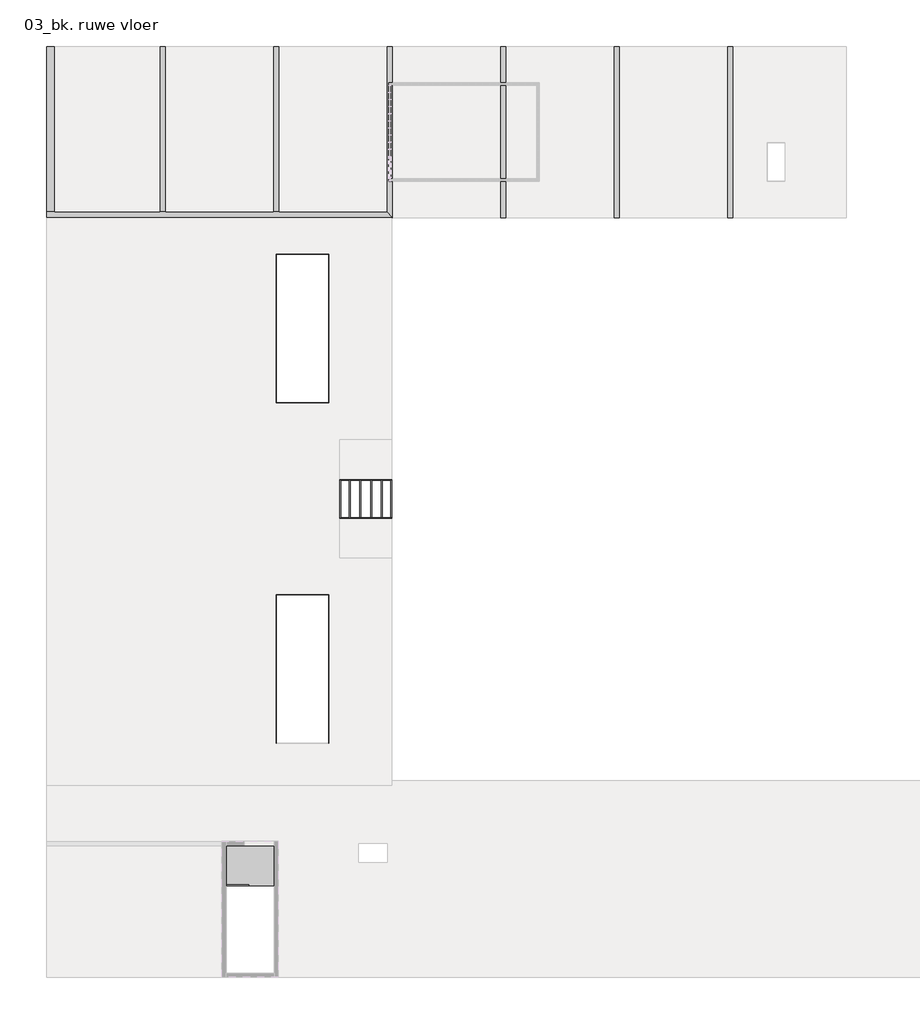
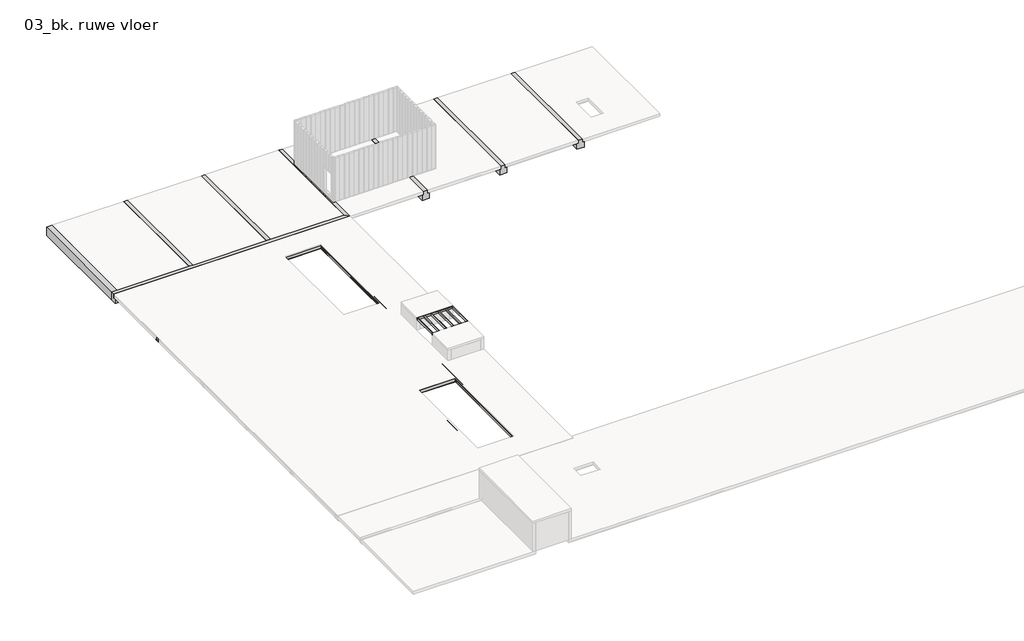
# One storey, part 9 of 9: 26 beams, 1 proxy.
"""IFC4 building model written with IfcOpenShell, lengths in millimetres."""

import ifcopenshell
import ifcopenshell.guid

model = None  # the IFC model being written
_history = None  # IfcOwnerHistory: only IFC2X3 demands one
_inside = {}  # id of a spatial element -> (the spatial element, [elements in it])
_under = {}  # id of a project, library or spatial element -> (it, [spatial elements below it])
_declared = {}  # id of a project -> (the project, [libraries it declares])
_typed = {}  # id of a type object -> (the type object, [elements of that type])
_made_of = {}  # id of a material, layer set ... -> (it, [elements and type objects made of it])


def new_model(schema):
    """Start an empty IFC model of exactly this schema.

    Asked for "IFC4X3", IfcOpenShell would pick the latest addendum, in which some entities
    have other attributes; the version numbers below select the first issue.
    IFC2X3 requires an IfcOwnerHistory on every rooted entity: one is made here for all.
    """
    global model, _history
    if schema == "IFC4X3":
        model = ifcopenshell.file(schema_version=(4, 3, 0, 0))
    else:
        model = ifcopenshell.file(schema=schema)
    _inside.clear()
    _under.clear()
    _declared.clear()
    _typed.clear()
    _made_of.clear()
    _history = None
    if model.schema == "IFC2X3":
        org = make("IfcOrganization", Name="unknown")
        user = make(
            "IfcPersonAndOrganization",
            ThePerson=make("IfcPerson", FamilyName="unknown"),
            TheOrganization=org,
        )
        app = make(
            "IfcApplication",
            ApplicationDeveloper=org,
            Version="unknown",
            ApplicationFullName="unknown",
            ApplicationIdentifier="unknown",
        )
        _history = make(
            "IfcOwnerHistory",
            OwningUser=user,
            OwningApplication=app,
            ChangeAction="ADDED",
            CreationDate=0,
        )
    return model


def make(cls, **values):
    """One entity of the class cls with the attributes given. An attribute that is None is left unset."""
    return model.create_entity(
        cls, **{name: value for name, value in values.items() if value is not None}
    )


def rooted(cls, **values):
    """An entity with a GlobalId (a new one), such as an element, a storey or a relation."""
    return make(cls, GlobalId=ifcopenshell.guid.new(), OwnerHistory=_history, **values)


def si_unit(unit_type, name, prefix=None):
    """IfcSIUnit, for example si_unit("LENGTHUNIT", "METRE", prefix="MILLI")."""
    return make("IfcSIUnit", UnitType=unit_type, Prefix=prefix, Name=name)


def assignment(units):
    """IfcUnitAssignment: the units of a project."""
    return None if units is None else make("IfcUnitAssignment", Units=units)


def point(xyz):
    """IfcCartesianPoint."""
    return None if xyz is None else make("IfcCartesianPoint", Coordinates=xyz)


def direction(xyz):
    """IfcDirection."""
    return None if xyz is None else make("IfcDirection", DirectionRatios=xyz)


def frame(location, z_axis=None, x_axis=None):
    """IfcAxis2Placement3D, a coordinate frame: its origin and axes. An axis left out is left unset."""
    return make(
        "IfcAxis2Placement3D",
        Location=point(location),
        Axis=direction(z_axis),
        RefDirection=direction(x_axis),
    )


def frame_2d(location, x_axis=None):
    """IfcAxis2Placement2D, a coordinate frame in the plane: its origin and x axis."""
    return make(
        "IfcAxis2Placement2D", Location=point(location), RefDirection=direction(x_axis)
    )


def origin():
    """The frame at (0, 0, 0) with its axes left unset."""
    return frame((0.0, 0.0, 0.0))


def place(relative_to, where):
    """IfcLocalPlacement: puts the frame where relative to a parent placement (None: the world)."""
    return make(
        "IfcLocalPlacement", PlacementRelTo=relative_to, RelativePlacement=where
    )


def context(
    kind, dimensions, precision=None, world=None, true_north=None, identifier=None
):
    """IfcGeometricRepresentationContext, for example the 3D "Model" context."""
    return make(
        "IfcGeometricRepresentationContext",
        ContextIdentifier=identifier,
        ContextType=kind,
        CoordinateSpaceDimension=dimensions,
        Precision=precision,
        WorldCoordinateSystem=world,
        TrueNorth=true_north,
    )


def project(units=None, contexts=None):
    """IfcProject with its units and contexts."""
    return rooted(
        "IfcProject",
        Name="project",
        RepresentationContexts=contexts,
        UnitsInContext=assignment(units),
    )


def spatial(cls, under=None, at=None, **own):
    """A site, building, storey or space (cls), placed at a placement, below another one or the project."""
    s = rooted(cls, ObjectPlacement=at, **own)
    if under is not None:
        _under.setdefault(under.id(), (under, []))[1].append(s)
    return s


def polyline(points):
    """IfcPolyline through the points."""
    return make("IfcPolyline", Points=[point(p) for p in points])


def circle_curve(where, radius):
    """IfcCircle in the frame where."""
    return make("IfcCircle", Position=where, Radius=radius)


def trimmed(basis, trim1, trim2, sense, master):
    """IfcTrimmedCurve: the piece of a basis curve between two trims."""
    return make(
        "IfcTrimmedCurve",
        BasisCurve=basis,
        Trim1=trim1,
        Trim2=trim2,
        SenseAgreement=sense,
        MasterRepresentation=master,
    )


def segment(curve, same_sense, transition):
    """IfcCompositeCurveSegment."""
    return make(
        "IfcCompositeCurveSegment",
        Transition=transition,
        SameSense=same_sense,
        ParentCurve=curve,
    )


def composite_curve(segments, self_intersect=None):
    """IfcCompositeCurve: segments joined end to end."""
    return make("IfcCompositeCurve", Segments=segments, SelfIntersect=self_intersect)


def outline(outer, holes=None, kind="AREA"):
    """IfcArbitraryClosedProfileDef: a profile drawn as a closed curve; with holes, ...WithVoids."""
    if holes is None:
        return make("IfcArbitraryClosedProfileDef", ProfileType=kind, OuterCurve=outer)
    return make(
        "IfcArbitraryProfileDefWithVoids",
        ProfileType=kind,
        OuterCurve=outer,
        InnerCurves=holes,
    )


def extrude(swept, where, along, depth):
    """IfcExtrudedAreaSolid: the profile swept, set in the frame where, extruded along a direction by depth."""
    return make(
        "IfcExtrudedAreaSolid",
        SweptArea=swept,
        Position=where,
        ExtrudedDirection=direction(along),
        Depth=depth,
    )


def faces_of(points, faces, orient=None, outer=None):
    """IfcFace entities. A face is a list of loops; a loop is a list of indices into points, from 0.

    orient and outer hold one flag for each loop. By default every Orientation is true, the
    first loop of a face is its IfcFaceOuterBound and the others are IfcFaceBound.
    """
    made = []
    for i, loops in enumerate(faces):
        bounds = []
        for j, loop in enumerate(loops):
            is_outer = j == 0 if outer is None else outer[i][j]
            bounds.append(
                make(
                    "IfcFaceOuterBound" if is_outer else "IfcFaceBound",
                    Bound=make("IfcPolyLoop", Polygon=[points[k] for k in loop]),
                    Orientation=True if orient is None else orient[i][j],
                )
            )
        made.append(make("IfcFace", Bounds=bounds))
    return made


def faceted_brep(points, faces, orient=None, outer=None, voids=None):
    """IfcFacetedBrep: a solid bounded by flat faces; with voids (closed shells), ...WithVoids."""
    shared = [point(p) for p in points]
    hull = make("IfcClosedShell", CfsFaces=faces_of(shared, faces, orient, outer))
    if voids is None:
        return make("IfcFacetedBrep", Outer=hull)
    return make(
        "IfcFacetedBrepWithVoids",
        Outer=hull,
        Voids=[
            make(cls, CfsFaces=faces_of(shared, fs, o, b)) for cls, fs, o, b in voids
        ],
    )


def shape(context_of_items, identifier, shape_type, items):
    """IfcShapeRepresentation: the items that make up one representation, for example the "Body"."""
    return make(
        "IfcShapeRepresentation",
        ContextOfItems=context_of_items,
        RepresentationIdentifier=identifier,
        RepresentationType=shape_type,
        Items=items,
    )


def source(mapping_origin, context_of_items, identifier, shape_type, items):
    """IfcRepresentationMap: a shape defined once, which mapped items show again and again."""
    return make(
        "IfcRepresentationMap",
        MappingOrigin=mapping_origin,
        MappedRepresentation=shape(context_of_items, identifier, shape_type, items),
    )


def transform(
    local_origin,
    x_axis=None,
    y_axis=None,
    z_axis=None,
    scale=None,
    scale2=None,
    scale3=None,
    uniform=True,
):
    """IfcCartesianTransformationOperator3D, or its non-uniform kind. x_axis, y_axis, z_axis: its Axis1, 2, 3."""
    if uniform:
        return make(
            "IfcCartesianTransformationOperator3D",
            Axis1=direction(x_axis),
            Axis2=direction(y_axis),
            LocalOrigin=point(local_origin),
            Scale=scale,
            Axis3=direction(z_axis),
        )
    return make(
        "IfcCartesianTransformationOperator3DnonUniform",
        Axis1=direction(x_axis),
        Axis2=direction(y_axis),
        LocalOrigin=point(local_origin),
        Scale=scale,
        Axis3=direction(z_axis),
        Scale2=scale2,
        Scale3=scale3,
    )


def mapped(mapping_source, mapping_target):
    """IfcMappedItem: shows the shape of a source again, moved by a transform."""
    return make(
        "IfcMappedItem", MappingSource=mapping_source, MappingTarget=mapping_target
    )


def made_of(thing, what):
    """Note that an element or type object is made of a material, layer set ...; save() writes the relation."""
    if what is not None:
        _made_of.setdefault(what.id(), (what, []))[1].append(thing)
    return thing


def element(
    cls,
    number,
    at=None,
    inside=None,
    cuts=None,
    type_object=None,
    material=None,
    context=None,
    identifier="Body",
    shape_type=None,
    held_by="IfcProductDefinitionShape",
    body=None,
    shapes=None,
    **own,
):
    """One element of the class cls, such as IfcWall. Its Tag is "e" and its number.

    at: its placement. inside: the storey or other place that contains it. cuts: it is an
    opening in that element (IfcRelVoidsElement). A single representation is given by context,
    identifier, shape_type and body (its items); several are given by shapes. held_by: the class
    of the entity that holds the representations. save() writes the other relations.
    """
    e = rooted(cls, Tag="e%d" % number, ObjectPlacement=at, **own)
    if body is not None:
        shapes = [shape(context, identifier, shape_type, body)]
    if shapes is not None:
        e.Representation = make(held_by, Representations=shapes)
    if inside is not None:
        _inside.setdefault(inside.id(), (inside, []))[1].append(e)
    if cuts is not None:
        rooted(
            "IfcRelVoidsElement", RelatingBuildingElement=cuts, RelatedOpeningElement=e
        )
    if type_object is not None:
        _typed.setdefault(type_object.id(), (type_object, []))[1].append(e)
    return made_of(e, material)


def aggregate(whole, parts):
    """IfcRelAggregates: a whole, such as a stair, and the parts it consists of."""
    return rooted("IfcRelAggregates", RelatingObject=whole, RelatedObjects=parts)


def save(model, path):
    """Write the relations noted so far, then the file.

    IfcRelAggregates (storeys below a building ...), IfcRelContainedInSpatialStructure (elements
    in a storey), IfcRelDefinesByType, IfcRelAssociatesMaterial and IfcRelDeclares: one each for
    every whole, place, type object, material and project.
    """
    for whole, parts in _under.values():
        aggregate(whole, parts)
    for where, things in _inside.values():
        rooted(
            "IfcRelContainedInSpatialStructure",
            RelatedElements=things,
            RelatingStructure=where,
        )
    for kind, things in _typed.values():
        rooted("IfcRelDefinesByType", RelatedObjects=things, RelatingType=kind)
    for what, things in _made_of.values():
        rooted("IfcRelAssociatesMaterial", RelatedObjects=things, RelatingMaterial=what)
    for by, libraries in _declared.values():
        rooted("IfcRelDeclares", RelatingContext=by, RelatedDefinitions=libraries)
    model.write(path)


def beam_736acf17(model_context):
    return source(origin(), model_context, "Body", "SweptSolid", [
        extrude(outline(polyline([(143.5, 280.0), (143.5, 0.0), (263.5, 0.0), (263.5, -20.0), (-286.5, -20.0), (-286.5, 0.0), (-166.5, 0.0), (-166.5, 280.0), (143.5, 280.0)]), holes=[polyline([(133.5, 0.0), (133.5, 250.0), (-156.5, 250.0), (-156.5, 0.0), (133.5, 0.0)])]), frame((-6445.0, 0.0, 0.0), z_axis=(1.0, 0.0, 0.0), x_axis=(0.0, 1.0, 0.0)), (0.0, 0.0, 1.0), 12890.0),
    ])


def beam_bc03ea60(model_context):
    return source(origin(), model_context, "Body", "SweptSolid", [
        extrude(outline(polyline([(-139.5, 280.0), (162.5, 280.0), (162.5, 0.0), (172.5, 0.0), (172.5, -15.0), (-277.5, -15.0), (-277.5, 0.0), (-139.5, 0.0), (-139.5, 280.0)]), holes=[polyline([(-133.5, 0.0), (156.5, 0.0), (156.5, 250.0), (-133.5, 250.0), (-133.5, 0.0)])]), frame((-1499.9999994, 0.0, 0.0), z_axis=(1.0, 0.0, 0.0), x_axis=(0.0, 1.0, 0.0)), (0.0, 0.0, 1.0), 2999.9999988),
    ])


def beam_09e22bfa(model_context):
    return source(origin(), model_context, "Body", "SweptSolid", [
        extrude(outline(polyline([(143.5, 280.0), (143.5, 0.0), (263.5, 0.0), (263.5, -20.0), (-286.5, -20.0), (-286.5, 0.0), (-166.5, 0.0), (-166.5, 280.0), (143.5, 280.0)]), holes=[polyline([(133.5, 0.0), (133.5, 250.0), (-156.5, 250.0), (-156.5, 0.0), (133.5, 0.0)])]), frame((-1682.5, 0.0, 0.0), z_axis=(1.0, 0.0, 0.0), x_axis=(0.0, 1.0, 0.0)), (0.0, 0.0, 1.0), 3365.0),
    ])


def beam_7c9e214b(model_context):
    return source(origin(), model_context, "Body", "SweptSolid", [
        extrude(outline(polyline([(139.5, 280.0), (139.5, 0.0), (277.5, 0.0), (277.5, -15.0), (-172.5, -15.0), (-172.5, 0.0), (-162.5, 0.0), (-162.5, 280.0), (139.5, 280.0)]), holes=[polyline([(133.5, 0.0), (133.5, 250.0), (-156.5, 250.0), (-156.5, 0.0), (133.5, 0.0)])]), frame((-1499.9999994, 0.0, 0.0), z_axis=(1.0, 0.0, 0.0), x_axis=(0.0, 1.0, 0.0)), (0.0, 0.0, 1.0), 2999.9999988),
    ])


def beam_87fc56b5(model_context):
    return source(origin(), model_context, "Body", "SweptSolid", [
        extrude(outline(polyline([(143.5, 280.0), (143.5, 0.0), (263.5, 0.0), (263.5, -20.0), (-286.5, -20.0), (-286.5, 0.0), (-166.5, 0.0), (-166.5, 280.0), (143.5, 280.0)]), holes=[polyline([(133.5, 0.0), (133.5, 250.0), (-156.5, 250.0), (-156.5, 0.0), (133.5, 0.0)])]), frame((-1812.5, 0.0, 0.0), z_axis=(1.0, 0.0, 0.0), x_axis=(0.0, 1.0, 0.0)), (0.0, 0.0, 1.0), 3365.0),
    ])


def beam_01d7d33a(model_context):
    return source(origin(), model_context, "Body", "SweptSolid", [
        extrude(outline(composite_curve([segment(polyline([(130.0, 112.5), (29.0, 112.5)]), True, "CONTINUOUS"), segment(trimmed(circle_curve(frame_2d((29.0, 88.5)), 24.0), [point((29.0, 112.5))], [point((5.0, 88.5))], True, "CARTESIAN"), True, "CONTINUOUS"), segment(polyline([(5.0, 88.5), (5.0, -88.5)]), True, "CONTINUOUS"), segment(trimmed(circle_curve(frame_2d((29.0, -88.5)), 24.0), [point((5.0, -88.5))], [point((29.0, -112.5))], True, "CARTESIAN"), True, "CONTINUOUS"), segment(polyline([(29.0, -112.5), (130.0, -112.5), (130.0, -130.0), (-130.0, -130.0), (-130.0, -112.5), (-29.0, -112.5)]), True, "CONTINUOUS"), segment(trimmed(circle_curve(frame_2d((-29.0, -88.5)), 24.0), [point((-29.0, -112.5))], [point((-5.0, -88.5))], True, "CARTESIAN"), True, "CONTINUOUS"), segment(polyline([(-5.0, -88.5), (-5.0, 88.5)]), True, "CONTINUOUS"), segment(trimmed(circle_curve(frame_2d((-29.0, 88.5)), 24.0), [point((-5.0, 88.5))], [point((-29.0, 112.5))], True, "CARTESIAN"), True, "CONTINUOUS"), segment(polyline([(-29.0, 112.5), (-130.0, 112.5), (-130.0, 130.0), (130.0, 130.0), (130.0, 112.5)]), True, "CONTINUOUS")], self_intersect=False)), frame((-6349.0, 0.0, 0.0), z_axis=(1.0, 0.0, 0.0), x_axis=(0.0, 1.0, 0.0)), (0.0, 0.0, 1.0), 12698.0),
    ])


def beam_3eaeb734(model_context):
    return source(origin(), model_context, "Body", "SweptSolid", [
        extrude(outline(composite_curve([segment(polyline([(-130.0, 112.5), (-130.0, 130.0), (130.0, 130.0), (130.0, 112.5), (29.0, 112.5)]), True, "CONTINUOUS"), segment(trimmed(circle_curve(frame_2d((29.0, 88.5)), 24.0), [point((29.0, 112.5))], [point((5.0, 88.5))], True, "CARTESIAN"), True, "CONTINUOUS"), segment(polyline([(5.0, 88.5), (5.0, -88.5)]), True, "CONTINUOUS"), segment(trimmed(circle_curve(frame_2d((29.0, -88.5)), 24.0), [point((5.0, -88.5))], [point((29.0, -112.5))], True, "CARTESIAN"), True, "CONTINUOUS"), segment(polyline([(29.0, -112.5), (130.0, -112.5), (130.0, -130.0), (-130.0, -130.0), (-130.0, -112.5), (-29.0, -112.5)]), True, "CONTINUOUS"), segment(trimmed(circle_curve(frame_2d((-29.0, -88.5)), 24.0), [point((-29.0, -112.5))], [point((-5.0, -88.5))], True, "CARTESIAN"), True, "CONTINUOUS"), segment(polyline([(-5.0, -88.5), (-5.0, 88.5)]), True, "CONTINUOUS"), segment(trimmed(circle_curve(frame_2d((-29.0, 88.5)), 24.0), [point((-5.0, 88.5))], [point((-29.0, 112.5))], True, "CARTESIAN"), True, "CONTINUOUS"), segment(polyline([(-29.0, 112.5), (-130.0, 112.5)]), True, "CONTINUOUS")], self_intersect=False)), frame((-6349.0, 0.0, 0.0), z_axis=(1.0, 0.0, 0.0), x_axis=(0.0, 1.0, 0.0)), (0.0, 0.0, 1.0), 12698.0),
    ])


def beam_0ced8335(model_context):
    return source(origin(), model_context, "Body", "SweptSolid", [
        extrude(outline(composite_curve([segment(polyline([(130.0, 112.5), (29.0, 112.5)]), True, "CONTINUOUS"), segment(trimmed(circle_curve(frame_2d((29.0, 88.5)), 24.0), [point((29.0, 112.5))], [point((5.0, 88.5))], True, "CARTESIAN"), True, "CONTINUOUS"), segment(polyline([(5.0, 88.5), (5.0, -88.5)]), True, "CONTINUOUS"), segment(trimmed(circle_curve(frame_2d((29.0, -88.5)), 24.0), [point((5.0, -88.5))], [point((29.0, -112.5))], True, "CARTESIAN"), True, "CONTINUOUS"), segment(polyline([(29.0, -112.5), (130.0, -112.5), (130.0, -130.0), (-130.0, -130.0), (-130.0, -112.5), (-29.0, -112.5)]), True, "CONTINUOUS"), segment(trimmed(circle_curve(frame_2d((-29.0, -88.5)), 24.0), [point((-29.0, -112.5))], [point((-5.0, -88.5))], True, "CARTESIAN"), True, "CONTINUOUS"), segment(polyline([(-5.0, -88.5), (-5.0, 88.5)]), True, "CONTINUOUS"), segment(trimmed(circle_curve(frame_2d((-29.0, 88.5)), 24.0), [point((-5.0, 88.5))], [point((-29.0, 112.5))], True, "CARTESIAN"), True, "CONTINUOUS"), segment(polyline([(-29.0, 112.5), (-130.0, 112.5), (-130.0, 130.0), (130.0, 130.0), (130.0, 112.5)]), True, "CONTINUOUS")], self_intersect=False)), frame((-6318.75, 0.0, 0.0), z_axis=(1.0, 0.0, 0.0), x_axis=(0.0, 1.0, 0.0)), (0.0, 0.0, 1.0), 12637.5),
    ])


def beam_f33d2ea4(model_context):
    return source(origin(), model_context, "Body", "SweptSolid", [
        extrude(outline(composite_curve([segment(polyline([(-130.0, 112.5), (-130.0, 130.0), (130.0, 130.0), (130.0, 112.5), (29.0, 112.5)]), True, "CONTINUOUS"), segment(trimmed(circle_curve(frame_2d((29.0, 88.5)), 24.0), [point((29.0, 112.5))], [point((5.0, 88.5))], True, "CARTESIAN"), True, "CONTINUOUS"), segment(polyline([(5.0, 88.5), (5.0, -88.5)]), True, "CONTINUOUS"), segment(trimmed(circle_curve(frame_2d((29.0, -88.5)), 24.0), [point((5.0, -88.5))], [point((29.0, -112.5))], True, "CARTESIAN"), True, "CONTINUOUS"), segment(polyline([(29.0, -112.5), (130.0, -112.5), (130.0, -130.0), (-130.0, -130.0), (-130.0, -112.5), (-29.0, -112.5)]), True, "CONTINUOUS"), segment(trimmed(circle_curve(frame_2d((-29.0, -88.5)), 24.0), [point((-29.0, -112.5))], [point((-5.0, -88.5))], True, "CARTESIAN"), True, "CONTINUOUS"), segment(polyline([(-5.0, -88.5), (-5.0, 88.5)]), True, "CONTINUOUS"), segment(trimmed(circle_curve(frame_2d((-29.0, 88.5)), 24.0), [point((-5.0, 88.5))], [point((-29.0, 112.5))], True, "CARTESIAN"), True, "CONTINUOUS"), segment(polyline([(-29.0, 112.5), (-130.0, 112.5)]), True, "CONTINUOUS")], self_intersect=False)), frame((-6318.75, 0.0, 0.0), z_axis=(1.0, 0.0, 0.0), x_axis=(0.0, 1.0, 0.0)), (0.0, 0.0, 1.0), 12637.5),
    ])


def beam_e7c6e874(model_context):
    return source(origin(), model_context, "Body", "SweptSolid", [
        extrude(outline(polyline([(-1067.0, -29.0), (-1067.0, 29.0), (1067.0, 29.0), (1067.0, -29.0), (-1067.0, -29.0)])), frame((0.0, 0.0, -78.0), z_axis=(0.0, 0.0, 1.0), x_axis=(1.0, 0.0, 0.0)), (0.0, 0.0, 1.0), 156.0),
    ])


def generic_models_f79be4d1(model_context):
    return source(origin(), model_context, "Body", "Brep", [
        faceted_brep([(1365.0, -2300.0, 0.0), (1365.0, -2300.0, -60.0), (1365.0, 0.0, -60.0), (1365.0, 0.0, 0.0), (-55.0, -2300.0, 0.0), (-55.0, -2190.0, 0.0), (-55.0, -2190.0, -110.0), (-55.0, -2300.0, -110.0), (-1365.0, 0.0, 0.0), (-1365.0, 0.0, -60.0), (-1365.0, -2190.0, -60.0), (-1365.0, -2190.0, 0.0), (-1335.0, -2300.0, -110.0), (-1335.0, -2300.0, -200.0), (-1210.0, -2300.0, -200.0), (-1210.0, -2300.0, -220.0), (1210.0, -2300.0, -220.0), (1210.0, -2300.0, -200.0), (1335.0, -2300.0, -200.0), (1335.0, -2300.0, -60.0), (-1335.0, -2190.0, -110.0), (-1335.0, -2190.0, -60.0), (1335.0, 0.0, -60.0), (1335.0, 0.0, -200.0), (1210.0, 0.0, -200.0), (1210.0, 0.0, -220.0), (-1210.0, 0.0, -220.0), (-1210.0, 0.0, -200.0), (-1335.0, 0.0, -200.0), (-1335.0, 0.0, -60.0)], [[[0, 1, 2, 3]], [[4, 5, 6, 7]], [[8, 9, 10, 11]], [[12, 13, 14, 15, 16, 17, 18, 19, 1, 0, 4, 7]], [[7, 6, 20, 12]], [[11, 10, 21, 20, 6, 5]], [[11, 5, 4, 0, 3, 8]], [[8, 3, 2, 22, 23, 24, 25, 26, 27, 28, 29, 9]], [[26, 25, 16, 15]], [[21, 10, 9, 29]], [[13, 12, 20, 21, 29, 28]], [[28, 27, 14, 13]], [[27, 26, 15, 14]], [[22, 2, 1, 19]], [[19, 18, 23, 22]], [[18, 17, 24, 23]], [[17, 16, 25, 24]]]),
    ])


model = new_model("IFC4")

# Units and contexts
model_context = context("Model", 3, world=origin())
ifc_project = project(units=[si_unit("LENGTHUNIT", "METRE", prefix="MILLI")], contexts=[model_context])

# Site, building, storey
site = spatial("IfcSite", under=ifc_project)
building = spatial("IfcBuilding", under=site)
storey = spatial("IfcBuildingStorey", under=building, Name="03_bk. ruwe vloer", Elevation=11330.0)

# Beams
placement = place(None, origin())
element("IfcBeam", 1, ObjectType="NLRS_28_SF_LIB_balk dubbele sponning beton prefab-CWV-MMBC-SRP_gen_rsf : balk beton prefab_gen__bxh 600x750 dubbele inkassing bxh 120x260", at=placement, inside=storey, context=model_context, shape_type="Brep", body=[
    faceted_brep([(32680.0, 43350.0, 11330.0), (32320.0, 43350.0, 11330.0), (32320.0, 43350.0, 11070.0), (32200.0, 43350.0, 11070.0), (32200.0, 43350.0, 10580.0), (32800.0, 43350.0, 10580.0), (32800.0, 43350.0, 11070.0), (32680.0, 43350.0, 11070.0), (32680.0, 53150.0, 11330.0), (32680.0, 53150.0, 11070.0), (32800.0, 53150.0, 11070.0), (32800.0, 53150.0, 10580.0), (32200.0, 53150.0, 10580.0), (32200.0, 53150.0, 11070.0), (32320.0, 53150.0, 11070.0), (32320.0, 53150.0, 11330.0), (32200.0, 53140.0, 11070.0), (32200.0, 43360.0, 11070.0), (32800.0, 53140.0, 11070.0), (32800.0, 43360.0, 11070.0)], [[[0, 1, 2, 3, 4, 5, 6, 7]], [[8, 9, 10, 11, 12, 13, 14, 15]], [[1, 0, 8, 15]], [[2, 1, 15, 14]], [[3, 2, 14, 13, 16, 17]], [[4, 3, 17, 16, 13, 12]], [[5, 4, 12, 11]], [[6, 5, 11, 10, 18, 19]], [[7, 6, 19, 18, 10, 9]], [[0, 7, 9, 8]]]),
])
element("IfcBeam", 2, ObjectType="NLRS_28_SF_LIB_balk dubbele sponning beton prefab-CWV-MMBC-SRP_gen_rsf : balk beton prefab_gen__bxh 600x750 dubbele inkassing bxh 120x260", at=placement, inside=storey, context=model_context, shape_type="Brep", body=[
    faceted_brep([(39180.0, 43350.0, 11330.0), (38820.0, 43350.0, 11330.0), (38820.0, 43350.0, 11070.0), (38700.0, 43350.0, 11070.0), (38700.0, 43350.0, 10580.0), (39300.0, 43350.0, 10580.0), (39300.0, 43350.0, 11070.0), (39180.0, 43350.0, 11070.0), (39180.0, 53150.0, 11330.0), (39180.0, 53150.0, 11070.0), (39300.0, 53150.0, 11070.0), (39300.0, 53150.0, 10580.0), (38700.0, 53150.0, 10580.0), (38700.0, 53150.0, 11070.0), (38820.0, 53150.0, 11070.0), (38820.0, 53150.0, 11330.0), (38700.0, 53140.0, 11070.0), (38700.0, 43360.0, 11070.0), (39300.0, 53140.0, 11070.0), (39300.0, 43360.0, 11070.0)], [[[0, 1, 2, 3, 4, 5, 6, 7]], [[8, 9, 10, 11, 12, 13, 14, 15]], [[1, 0, 8, 15]], [[2, 1, 15, 14]], [[3, 2, 14, 13, 16, 17]], [[4, 3, 17, 16, 13, 12]], [[5, 4, 12, 11]], [[6, 5, 11, 10, 18, 19]], [[7, 6, 19, 18, 10, 9]], [[0, 7, 9, 8]]]),
])
element("IfcBeam", 3, ObjectType="NLRS_28_SF_LIB_balk dubbele sponning beton prefab-CWV-MMBC-SRP_gen_rsf : balk beton prefab_gen__bxh 600x750 dubbele inkassing bxh 120x260", at=placement, inside=storey, context=model_context, shape_type="Brep", body=[
    faceted_brep([(45680.0, 43350.0, 11330.0), (45320.0, 43350.0, 11330.0), (45320.0, 43350.0, 11070.0), (45200.0, 43350.0, 11070.0), (45200.0, 43350.0, 10580.0), (45800.0, 43350.0, 10580.0), (45800.0, 43350.0, 11070.0), (45680.0, 43350.0, 11070.0), (45680.0, 53150.0, 11330.0), (45680.0, 53150.0, 11070.0), (45800.0, 53150.0, 11070.0), (45800.0, 53150.0, 10580.0), (45200.0, 53150.0, 10580.0), (45200.0, 53150.0, 11070.0), (45320.0, 53150.0, 11070.0), (45320.0, 53150.0, 11330.0), (45200.0, 53140.0, 11070.0), (45200.0, 43360.0, 11070.0), (45800.0, 53140.0, 11070.0), (45800.0, 43360.0, 11070.0)], [[[0, 1, 2, 3, 4, 5, 6, 7]], [[8, 9, 10, 11, 12, 13, 14, 15]], [[1, 0, 8, 15]], [[2, 1, 15, 14]], [[3, 2, 14, 13, 16, 17]], [[4, 3, 17, 16, 13, 12]], [[5, 4, 12, 11]], [[6, 5, 11, 10, 18, 19]], [[7, 6, 19, 18, 10, 9]], [[0, 7, 9, 8]]]),
])
element("IfcBeam", 4, ObjectType="NLRS_28_SF_LIB_balk dubbele sponning beton prefab-CWV-MMBC-SRP_gen_rsf : balk beton prefab_gen__bxh 600x750 dubbele inkassing bxh 120x260", at=placement, inside=storey, context=model_context, shape_type="Brep", body=[
    faceted_brep([(26180.0, 53150.0, 11330.0), (26180.0, 53150.0, 11070.0), (26300.0, 53150.0, 11070.0), (26300.0, 53150.0, 10580.0), (25700.0, 53150.0, 10580.0), (25700.0, 53150.0, 11070.0), (25820.0, 53150.0, 11070.0), (25820.0, 53150.0, 11330.0), (25820.0, 43680.0, 11330.0), (26150.0, 43350.0, 11330.0), (26180.0, 43350.0, 11330.0), (25820.0, 43680.0, 11070.0), (25700.0, 53140.0, 11070.0), (25700.0, 43800.0, 11070.0), (25725.0, 43775.0, 11070.0), (25700.0, 43800.0, 10580.0), (26300.0, 43350.0, 10580.0), (26150.0, 43350.0, 10580.0), (26300.0, 53140.0, 11070.0), (26300.0, 43360.0, 11070.0), (26300.0, 43350.0, 11070.0), (26180.0, 43350.0, 11070.0)], [[[0, 1, 2, 3, 4, 5, 6, 7]], [[0, 7, 8, 9, 10]], [[7, 6, 11, 8]], [[6, 5, 12, 13, 14, 11]], [[5, 4, 15, 13, 12]], [[4, 3, 16, 17, 15]], [[3, 2, 18, 19, 20, 16]], [[2, 1, 21, 20, 19, 18]], [[1, 0, 10, 21]], [[8, 11, 14, 13, 15, 17, 9]], [[17, 16, 20, 21, 10, 9]]]),
])
element("IfcBeam", 5, ObjectType="NLRS_28_SF_LIB_balk dubbele sponning beton prefab-CWV-MMBC-SRP_gen_rsf : balk beton prefab_gen__bxh 600x750 dubbele inkassing bxh 120x260", at=placement, inside=storey, context=model_context, shape_type="Brep", body=[
    faceted_brep([(19680.0, 53150.0, 11330.0), (19680.0, 53150.0, 11070.0), (19800.0, 53150.0, 11070.0), (19800.0, 53150.0, 10580.0), (19200.0, 53150.0, 10580.0), (19200.0, 53150.0, 11070.0), (19320.0, 53150.0, 11070.0), (19320.0, 53150.0, 11330.0), (19320.0, 43680.0, 11330.0), (19680.0, 43680.0, 11330.0), (19320.0, 43800.0, 11070.0), (19320.0, 43680.0, 11070.0), (19200.0, 53140.0, 11070.0), (19200.0, 43800.0, 11070.0), (19225.0, 43800.0, 11070.0), (19200.0, 43800.0, 10580.0), (19800.0, 43800.0, 10580.0), (19800.0, 53140.0, 11070.0), (19800.0, 43800.0, 11070.0), (19680.0, 43800.0, 11070.0), (19775.0, 43800.0, 11070.0), (19680.0, 43680.0, 11070.0)], [[[0, 1, 2, 3, 4, 5, 6, 7]], [[0, 7, 8, 9]], [[7, 6, 10, 11, 8]], [[6, 5, 12, 13, 14, 10]], [[5, 4, 15, 13, 12]], [[4, 3, 16, 15]], [[3, 2, 17, 18, 16]], [[2, 1, 19, 20, 18, 17]], [[1, 0, 9, 21, 19]], [[19, 10, 14, 13, 15, 16, 18, 20]], [[21, 11, 10, 19]], [[11, 21, 9, 8]]]),
])
element("IfcBeam", 6, ObjectType="NLRS_28_SF_LIB_balk dubbele sponning beton prefab-CWV-MMBC-SRP_gen_rsf : balk beton prefab_gen__bxh 600x750 dubbele inkassing bxh 120x260", at=placement, inside=storey, context=model_context, shape_type="Brep", body=[
    faceted_brep([(13180.0, 53150.0, 11330.0), (13180.0, 53150.0, 11070.0), (13300.0, 53150.0, 11070.0), (13300.0, 53150.0, 10580.0), (12700.0, 53150.0, 10580.0), (12700.0, 53150.0, 11070.0), (12820.0, 53150.0, 11070.0), (12820.0, 53150.0, 11330.0), (12820.0, 43680.0, 11330.0), (13180.0, 43680.0, 11330.0), (12820.0, 43800.0, 11070.0), (12820.0, 43680.0, 11070.0), (12700.0, 53140.0, 11070.0), (12700.0, 43800.0, 11070.0), (12700.0, 43800.0, 10580.0), (13300.0, 43800.0, 10580.0), (13300.0, 53140.0, 11070.0), (13300.0, 43800.0, 11070.0), (13180.0, 43800.0, 11070.0), (13180.0, 43680.0, 11070.0)], [[[0, 1, 2, 3, 4, 5, 6, 7]], [[0, 7, 8, 9]], [[7, 6, 10, 11, 8]], [[6, 5, 12, 13, 10]], [[5, 4, 14, 13, 12]], [[4, 3, 15, 14]], [[3, 2, 16, 17, 15]], [[2, 1, 18, 17, 16]], [[1, 0, 9, 19, 18]], [[18, 10, 13, 14, 15, 17]], [[19, 11, 10, 18]], [[11, 19, 9, 8]]]),
])
element("IfcBeam", 7, ObjectType="NLRS_28_SF_LIB_balk enkele sponning beton prefab-CWV-MMBC-SRP_gen_rsf : balk beton prefab_gen__bxh 600x750 met inkassing bxh120x260", at=placement, inside=storey, context=model_context, shape_type="Brep", body=[
    faceted_brep([(6350.0, 43680.0, 11330.0), (6350.0, 43680.0, 10580.0), (6950.0, 43680.0, 10580.0), (6950.0, 43680.0, 11070.0), (6830.0, 43680.0, 11070.0), (6830.0, 43680.0, 11330.0), (6350.0, 53150.0, 11330.0), (6830.0, 53150.0, 11330.0), (6830.0, 53150.0, 11070.0), (6950.0, 53150.0, 11070.0), (6950.0, 53150.0, 10580.0), (6350.0, 53150.0, 10580.0), (6950.0, 43775.0, 11070.0), (6950.0, 43800.0, 11070.0), (6950.0, 53140.0, 11070.0), (6950.0, 43800.0, 10580.0)], [[[0, 1, 2, 3, 4, 5]], [[6, 7, 8, 9, 10, 11]], [[0, 5, 7, 6]], [[5, 4, 8, 7]], [[4, 3, 12, 13, 14, 9, 8]], [[3, 2, 15, 10, 9, 14, 13, 12]], [[2, 1, 11, 10, 15]], [[1, 0, 6, 11]]]),
])
element("IfcBeam", 8, ObjectType="NLRS_28_SF_LIB_balk dubbele sponning beton prefab-CWV-MMBC-SRP_gen_rsf : balk beton prefab_gen__bxh 600x750 dubbele inkassing bxh 120x260 en 150x330", at=placement, inside=storey, context=model_context, shape_type="Brep", body=[
    faceted_brep([(6350.0, 43350.0, 11330.0), (6350.0, 43680.0, 11330.0), (6350.0, 43680.0, 10580.0), (6350.0, 43200.0, 10580.0), (6350.0, 43200.0, 11000.0), (6350.0, 43330.0, 11000.0), (6350.0, 43350.0, 11000.0), (6350.0, 43350.0, 11260.0), (26125.0, 43350.0, 11330.0), (26150.0, 43350.0, 11330.0), (25820.0, 43680.0, 11330.0), (19680.0, 43680.0, 11330.0), (19320.0, 43680.0, 11330.0), (13180.0, 43680.0, 11330.0), (12820.0, 43680.0, 11330.0), (6830.0, 43680.0, 11330.0), (26125.0, 43350.0, 11000.0), (26125.0, 43350.0, 10580.0), (26150.0, 43350.0, 10580.0), (19240.0, 43200.0, 11000.0), (19500.0, 43200.0, 11000.0), (22500.0, 43200.0, 11000.0), (22760.0, 43200.0, 11000.0), (26125.0, 43200.0, 11000.0), (26125.0, 43330.0, 11000.0), (26125.0, 43200.0, 10580.0), (25700.0, 43800.0, 10580.0), (6950.0, 43680.0, 10580.0), (6950.0, 43800.0, 10580.0), (12700.0, 43800.0, 10580.0), (13300.0, 43800.0, 10580.0), (19200.0, 43800.0, 10580.0), (19800.0, 43800.0, 10580.0), (25700.0, 43800.0, 11070.0), (6950.0, 43800.0, 11070.0), (12700.0, 43800.0, 11070.0), (12725.0, 43800.0, 11070.0), (12820.0, 43800.0, 11070.0), (13180.0, 43800.0, 11070.0), (13275.0, 43800.0, 11070.0), (13300.0, 43800.0, 11070.0), (19200.0, 43800.0, 11070.0), (19225.0, 43800.0, 11070.0), (19320.0, 43800.0, 11070.0), (19680.0, 43800.0, 11070.0), (19775.0, 43800.0, 11070.0), (19800.0, 43800.0, 11070.0), (25820.0, 43680.0, 11070.0), (25725.0, 43775.0, 11070.0), (6950.0, 43775.0, 11070.0), (6950.0, 43680.0, 11070.0), (12820.0, 43680.0, 11070.0), (13180.0, 43680.0, 11070.0), (19320.0, 43680.0, 11070.0), (19680.0, 43680.0, 11070.0)], [[[0, 1, 2, 3, 4, 5, 6, 7]], [[1, 0, 8, 9, 10, 11, 12, 13, 14, 15]], [[6, 16, 17, 18, 9, 8, 0, 7]], [[16, 6, 5, 4, 19, 20, 21, 22, 23, 24]], [[4, 3, 25, 23, 22, 21, 20, 19]], [[26, 18, 17, 25, 3, 2, 27, 28, 29, 30, 31, 32]], [[33, 26, 32, 31, 30, 29, 28, 34, 35, 36, 37, 38, 39, 40, 41, 42, 43, 44, 45, 46]], [[47, 48, 33, 46, 45, 44, 43, 42, 41, 40, 39, 38, 37, 36, 35, 34, 49, 50, 51, 52, 53, 54]], [[10, 47, 54, 53, 52, 51, 50, 27, 2, 1, 15, 14, 13, 12, 11]], [[10, 9, 18, 26, 33, 48, 47]], [[34, 28, 27, 50, 49]], [[17, 16, 24, 23, 25]]]),
])
element("IfcBeam", 9, ObjectType="NLRS_28_SF_LIB_houten balk-MMBW-SRP_gen_rsf : houten balk_gen__bxh 58x156", at=placement, inside=storey, context=model_context, shape_type="SweptSolid", body=[
    extrude(outline(polyline([(26125.0, 26183.0), (26067.0, 26183.0), (26067.0, 28317.0), (26125.0, 28317.0), (26125.0, 26183.0)])), frame((0.0, 0.0, 12276.0), z_axis=(0.0, 0.0, 1.0), x_axis=(1.0, 0.0, 0.0)), (0.0, 0.0, 1.0), 156.0),
])
element("IfcBeam", 10, ObjectType="NLRS_28_SF_LIB_houten balk-MMBW-SRP_gen_rsf : houten balk_gen__bxh 58x156", at=placement, inside=storey, context=model_context, shape_type="SweptSolid", body=[
    extrude(outline(polyline([(23183.0, 26183.0), (23125.0, 26183.0), (23125.0, 28317.0), (23183.0, 28317.0), (23183.0, 26183.0)])), frame((0.0, 0.0, 12276.0), z_axis=(0.0, 0.0, 1.0), x_axis=(1.0, 0.0, 0.0)), (0.0, 0.0, 1.0), 156.0),
])
element("IfcBeam", 11, ObjectType="NLRS_28_SF_LIB_houten balk-MMBW-SRP_gen_rsf : houten balk_gen__bxh 58x156", at=placement, inside=storey, context=model_context, shape_type="SweptSolid", body=[
    extrude(outline(polyline([(23125.0, 28317.0), (23125.0, 28375.0), (26125.0, 28375.0), (26125.0, 28317.0), (23125.0, 28317.0)])), frame((0.0, 0.0, 12276.0), z_axis=(0.0, 0.0, 1.0), x_axis=(1.0, 0.0, 0.0)), (0.0, 0.0, 1.0), 156.0),
])
element("IfcBeam", 12, ObjectType="NLRS_28_SF_LIB_houten balk-MMBW-SRP_gen_rsf : houten balk_gen__bxh 58x156", at=placement, inside=storey, context=model_context, shape_type="SweptSolid", body=[
    extrude(outline(polyline([(23125.0, 26183.0), (26125.0, 26183.0), (26125.0, 26125.0), (23125.0, 26125.0), (23125.0, 26183.0)])), frame((0.0, 0.0, 12276.0), z_axis=(0.0, 0.0, 1.0), x_axis=(1.0, 0.0, 0.0)), (0.0, 0.0, 1.0), 156.0),
])
beam_shape = beam_736acf17(model_context)
element("IfcBeam", 13, ObjectType="NLRS_28_SF_LIB_stalen ligger THQ-AV-CWV-MMBS-SRP_gen_rsf : stalen ligger_gen__THQ_280x10-290x30-550x20", at=placement, inside=storey, context=model_context, shape_type="MappedRepresentation", body=[
    mapped(beam_shape, transform((12795.0, 36988.5, 11000.0), x_axis=(-1.0, 0.0, 0.0), y_axis=(0.0, -1.0, 0.0), z_axis=(0.0, 0.0, 1.0))),
])
beam_2_shape = beam_bc03ea60(model_context)
element("IfcBeam", 14, ObjectType="NLRS_28_SF_LIB_stalen ligger THQ-AV-CWV-MMBS-SRP_gen_rsf : stalen ligger_gen__PET 280x6-290x30-450x15", at=placement, inside=storey, context=model_context, shape_type="MappedRepresentation", body=[
    mapped(beam_2_shape, transform((21000.0, 21922.5, 11000.0), x_axis=(-1.0, 0.0, 0.0), y_axis=(0.0, -1.0, 0.0), z_axis=(0.0, 0.0, 1.0))),
])
element("IfcBeam", 15, ObjectType="NLRS_28_SF_LIB_stalen ligger THQ-AV-CWV-MMBS-SRP_gen_rsf : stalen ligger_gen__PET 280x6-290x30-450x15", at=placement, inside=storey, context=model_context, shape_type="MappedRepresentation", body=[
    mapped(beam_2_shape, transform((21000.0, 41422.5, 11000.0), x_axis=(-1.0, 0.0, 0.0), y_axis=(0.0, -1.0, 0.0), z_axis=(0.0, 0.0, 1.0))),
])
beam_3_shape = beam_09e22bfa(model_context)
element("IfcBeam", 16, ObjectType="NLRS_28_SF_LIB_stalen ligger THQ-AV-CWV-MMBS-SRP_gen_rsf : stalen ligger_gen__THQ_280x10-290x30-550x20", at=placement, inside=storey, context=model_context, shape_type="MappedRepresentation", body=[
    mapped(beam_3_shape, transform((24442.5, 36988.5, 11000.0), x_axis=(-1.0, 0.0, 0.0), y_axis=(0.0, -1.0, 0.0), z_axis=(0.0, 0.0, 1.0))),
])
beam_4_shape = beam_7c9e214b(model_context)
element("IfcBeam", 17, ObjectType="NLRS_28_SF_LIB_stalen ligger THQ-AV-CWV-MMBS-SRP_gen_rsf : stalen ligger_gen__PET 280x6-290x30-450x15", at=placement, inside=storey, context=model_context, shape_type="MappedRepresentation", body=[
    mapped(beam_4_shape, transform((21000.0, 32577.5, 11000.0), x_axis=(-1.0, 0.0, 0.0), y_axis=(0.0, -1.0, 0.0), z_axis=(0.0, 0.0, 1.0))),
])
beam_5_shape = beam_87fc56b5(model_context)
element("IfcBeam", 18, ObjectType="NLRS_28_SF_LIB_stalen ligger THQ-AV-CWV-MMBS-SRP_gen_rsf : stalen ligger_gen__THQ_280x10-290x30-550x20", at=placement, inside=storey, context=model_context, shape_type="MappedRepresentation", body=[
    mapped(beam_5_shape, transform((24312.5, 17488.5, 11000.0), x_axis=(-1.0, 0.0, 0.0), y_axis=(0.0, -1.0, 0.0), z_axis=(0.0, 0.0, 1.0))),
])
beam_6_shape = beam_01d7d33a(model_context)
element("IfcBeam", 19, ObjectType="NLRS_28_SF_LIB_stalen ligger HEB-AV-CWV-MMBS-SRP_gen_rsf : stalen ligger_gen__HEB 260", at=placement, inside=storey, context=model_context, shape_type="MappedRepresentation", body=[
    mapped(beam_6_shape, transform((19370.0, 17511.5, 11130.0), x_axis=(0.0, -1.0, 0.0), y_axis=(1.0, 0.0, 0.0), z_axis=(0.0, 0.0, 1.0))),
])
beam_7_shape = beam_3eaeb734(model_context)
element("IfcBeam", 20, ObjectType="NLRS_28_SF_LIB_stalen ligger HEB-AV-CWV-MMBS-SRP_gen_rsf : stalen ligger_gen__HEB 260", at=placement, inside=storey, context=model_context, shape_type="MappedRepresentation", body=[
    mapped(beam_7_shape, transform((22630.0, 17511.5, 11130.0), x_axis=(0.0, -1.0, 0.0), y_axis=(1.0, 0.0, 0.0), z_axis=(0.0, 0.0, 1.0))),
])
beam_8_shape = beam_0ced8335(model_context)
element("IfcBeam", 21, ObjectType="NLRS_28_SF_LIB_stalen ligger HEB-AV-CWV-MMBS-SRP_gen_rsf : stalen ligger_gen__HEB 260", at=placement, inside=storey, context=model_context, shape_type="MappedRepresentation", body=[
    mapped(beam_8_shape, transform((19370.0, 36981.25, 11130.0), x_axis=(0.0, -1.0, 0.0), y_axis=(1.0, 0.0, 0.0), z_axis=(0.0, 0.0, 1.0))),
])
beam_9_shape = beam_f33d2ea4(model_context)
element("IfcBeam", 22, ObjectType="NLRS_28_SF_LIB_stalen ligger HEB-AV-CWV-MMBS-SRP_gen_rsf : stalen ligger_gen__HEB 260", at=placement, inside=storey, context=model_context, shape_type="MappedRepresentation", body=[
    mapped(beam_9_shape, transform((22630.0, 36981.25, 11130.0), x_axis=(0.0, -1.0, 0.0), y_axis=(1.0, 0.0, 0.0), z_axis=(0.0, 0.0, 1.0))),
])
beam_10_shape = beam_e7c6e874(model_context)
element("IfcBeam", 23, ObjectType="NLRS_28_SF_LIB_houten balk-MMBW-SRP_gen_rsf : houten balk_gen__bxh 58x156", at=placement, inside=storey, context=model_context, shape_type="MappedRepresentation", body=[
    mapped(beam_10_shape, transform((24930.0, 27250.0, 12354.0), x_axis=(0.0, 1.0, 0.0), y_axis=(-1.0, 0.0, 0.0), z_axis=(0.0, 0.0, 1.0))),
])
element("IfcBeam", 24, ObjectType="NLRS_28_SF_LIB_houten balk-MMBW-SRP_gen_rsf : houten balk_gen__bxh 58x156", at=placement, inside=storey, context=model_context, shape_type="MappedRepresentation", body=[
    mapped(beam_10_shape, transform((24320.0, 27250.0, 12354.0), x_axis=(0.0, 1.0, 0.0), y_axis=(-1.0, 0.0, 0.0), z_axis=(0.0, 0.0, 1.0))),
])
element("IfcBeam", 25, ObjectType="NLRS_28_SF_LIB_houten balk-MMBW-SRP_gen_rsf : houten balk_gen__bxh 58x156", at=placement, inside=storey, context=model_context, shape_type="MappedRepresentation", body=[
    mapped(beam_10_shape, transform((23710.0, 27250.0, 12354.0), x_axis=(0.0, 1.0, 0.0), y_axis=(-1.0, 0.0, 0.0), z_axis=(0.0, 0.0, 1.0))),
])
element("IfcBeam", 26, ObjectType="NLRS_28_SF_LIB_houten balk-MMBW-SRP_gen_rsf : houten balk_gen__bxh 58x156", at=placement, inside=storey, context=model_context, shape_type="MappedRepresentation", body=[
    mapped(beam_10_shape, transform((25540.0, 27250.0, 12354.0), x_axis=(0.0, 1.0, 0.0), y_axis=(-1.0, 0.0, 0.0), z_axis=(0.0, 0.0, 1.0))),
])

# Proxy
generic_models_shape = generic_models_f79be4d1(model_context)
element("IfcBuildingElementProxy", 27, Name="NLRS_24_GM_UN_rechthoekig bordes prefab zonder oplegnok-AV_gen_rsf : prefab bordes_gen__2300x2730", ObjectType="NLRS_24_GM_UN_rechthoekig bordes prefab zonder oplegnok-AV_gen_rsf : prefab bordes_gen__2300x2730", at=placement, inside=storey, context=model_context, shape_type="MappedRepresentation", body=[
    mapped(generic_models_shape, transform((18000.0, 7390.0, 11400.0), x_axis=(1.0, 0.0, 0.0), y_axis=(0.0, 1.0, 0.0), z_axis=(0.0, 0.0, 1.0))),
])

save(model, "model.ifc")

# Revit data of these elements
# Type "NLRS_28_SF_LIB_balk dubbele sponning beton prefab-CWV-MMBC-SRP_gen_rsf : balk beton prefab_gen__bxh 600x750 dubbele inkassing bxh 120x260"
#   Export Type to IFC As = "IfcBeamType"
#   Type IfcGUID = "0AFZSao6j3uApvehgmz3fk"
#   Type Comments = "600x750"
#   Description = "balk beton ihwg 600x750 dubbele inkassing 120x260"
#   Assembly Code = "28.11"
#   RSF_C_hoogte_inkassing_rechts = 260 mm
#   RSF_C_hoogte_inkassing_links = 260 mm
#   RSF_C_breedte_inkassing_rechts = 120 mm
#   RSF_C_breedte_inkassing_links = 120 mm
#   NLRS_C_lengte [instance default] = 3000 mm
#   NLRS_C_hoogte = 750 mm
#   NLRS_C_breedte = 600 mm
#   Length [instance default] = 3000 mm
#   Structural Material = NLRS_f2_beton prefab_gen_rsf
#   Model = ""
# Type "NLRS_28_SF_LIB_balk enkele sponning beton prefab-CWV-MMBC-SRP_gen_rsf : balk beton prefab_gen__bxh 600x750 met inkassing bxh120x260"
#   Export Type to IFC As = "IfcBeamType"
#   Type IfcGUID = "3_OCAr9yj6mwah3L5tr_yL"
#   Type Comments = "600x750"
#   Description = "balk beton ihwg 600x750 inkassing 120x260"
#   Assembly Code = "28.11"
#   RSF_C_hoogte_inkassing_rechts = 260 mm
#   RSF_C_breedte_inkassing_rechts = 120 mm
#   NLRS_C_lengte [instance default] = 3000 mm
#   NLRS_C_hoogte = 750 mm
#   NLRS_C_breedte = 600 mm
#   Length [instance default] = 3000 mm
#   Structural Material = NLRS_f2_beton prefab_gen_rsf
#   Model = ""
# Type "NLRS_28_SF_LIB_balk dubbele sponning beton prefab-CWV-MMBC-SRP_gen_rsf : balk beton prefab_gen__bxh 600x750 dubbele inkassing bxh 120x260 en 150x330"
#   Export Type to IFC As = "IfcBeamType"
#   Type IfcGUID = "13lTCcCQ95UOWcvnmPh7X3"
#   Type Comments = "600x750"
#   Description = "balk beton ihwg 600x750 dubbele inkassing 120x260 en 150x330"
#   Assembly Code = "28.11"
#   RSF_C_hoogte_inkassing_rechts = 330 mm
#   RSF_C_hoogte_inkassing_links = 260 mm
#   RSF_C_breedte_inkassing_rechts = 150 mm
#   RSF_C_breedte_inkassing_links = 120 mm
#   NLRS_C_lengte [instance default] = 3000 mm
#   NLRS_C_hoogte = 750 mm
#   NLRS_C_breedte = 600 mm
#   Length [instance default] = 3000 mm
#   Structural Material = NLRS_f2_beton prefab_gen_rsf
#   Model = ""
# Type "NLRS_28_SF_LIB_houten balk-MMBW-SRP_gen_rsf : houten balk_gen__bxh 58x156"
#   Export Type to IFC As = "IfcBeamType"
#   Type IfcGUID = "07M7mRoiH1CR8m_RSKIvXg"
#   Type Comments = "58x156"
#   Model = " "
#   Manufacturer = " "
#   Fire Rating = " "
#   Description = "houten balk 58x156"
#   Assembly Code = "28.11"
#   NLRS_C_lengte [instance default] = 3000 mm
#   NLRS_C_hoogte = 156 mm
#   NLRS_C_breedte = 58 mm
#   Length [instance default] = 3000 mm
#   Structural Material = NLRS_i2_hout naaldhout vuren_gen_rsf
#   Keynote = ""
# Type "NLRS_28_SF_LIB_stalen ligger THQ-AV-CWV-MMBS-SRP_gen_rsf : stalen ligger_gen__THQ_280x10-290x30-550x20"
#   Export Type to IFC As = "IfcBeamType"
#   Type IfcGUID = "2GRbcre991teoKeCLB8MAm"
#   Type Comments = "THQ 280x10-290x30-550x20"
#   Model = " "
#   Manufacturer = " "
#   Fire Rating = " "
#   Description = "stalen ligger THQ 280x10-290x30-550x20"
#   Assembly Code = "28.11"
#   tw = 10 mm
#   tu = 20 mm
#   to = 30 mm
#   h = 280 mm
#   bu = 550 mm
#   bo = 290 mm
#   NLRS_C_lengte [instance default] = 1500 mm
#   Length [instance default] = 1500 mm
#   RSF_C_vullen_met_beton [instance default] = no
#   RSF_C_petligger = no
#   RSF_C_hoedligger = yes
#   Structural Material = NLRS_h2_staal_gen_rsf
#   Keynote = ""
# Type "NLRS_28_SF_LIB_stalen ligger THQ-AV-CWV-MMBS-SRP_gen_rsf : stalen ligger_gen__PET 280x6-290x30-450x15"
#   Export Type to IFC As = "IfcBeamType"
#   Type IfcGUID = "0zo1UjqZ91lRsfCKsOOaAF"
#   Type Comments = "PET 280x6-290x30-450x15"
#   Model = " "
#   Manufacturer = " "
#   Fire Rating = " "
#   Description = "stalen ligger PET 280x6-290x30-450x15"
#   Assembly Code = "28.11"
#   tw = 6 mm
#   tu = 15 mm
#   to = 30 mm
#   h = 280 mm
#   bu = 450 mm
#   bo = 290 mm
#   NLRS_C_lengte [instance default] = 1500 mm
#   Length [instance default] = 1500 mm
#   RSF_C_vullen_met_beton [instance default] = no
#   RSF_C_petligger = yes
#   RSF_C_hoedligger = no
#   Structural Material = NLRS_h2_staal_gen_rsf
#   Keynote = ""
# Type "NLRS_28_SF_LIB_stalen ligger HEB-AV-CWV-MMBS-SRP_gen_rsf : stalen ligger_gen__HEB 260"
#   Export Type to IFC As = "IfcBeamType"
#   Type IfcGUID = "0zo1UjqZ91lRsfCKsOOa5a"
#   Type Comments = "HEB260"
#   Model = " "
#   Manufacturer = " "
#   Fire Rating = " "
#   Description = "stalen ligger HEB260"
#   Assembly Code = "28.11"
#   ra = 24 mm
#   vz = 130 mm
#   vy = 130 mm
#   vpz = 130 mm
#   vpy = 130 mm
#   NLRS_C_lengte [instance default] = 1500 mm
#   Length [instance default] = 1500 mm
#   bf = 260 mm
#   d = 260 mm
#   tf = 17.5 mm
#   tw = 10 mm
#   Structural Material = NLRS_h2_staal_gen_rsf
#   Keynote = ""
# Type "NLRS_24_GM_UN_rechthoekig bordes prefab zonder oplegnok-AV_gen_rsf : prefab bordes_gen__2300x2730"
#   Export Type to IFC As = "IfcStair"
#   Type IfcGUID = "2CEqVLPNH8KRN7ghwV3a_c"
#   Type Comments = " "
#   Model = " "
#   Manufacturer = " "
#   Description = "rechthoekig bordes prefab\r\n1930x4395"
#   Assembly Code = "24.15"
#   Width = 2730 mm
#   Thickness = 220 mm
#   Perimeter = 10060 mm
#   NLRS_C_lengte_02 = 1310 mm
#   NLRS_C_lengte_01 = 1310 mm
#   NLRS_C_hoogte_02 = 110 mm
#   NLRS_C_hoogte_01 = 110 mm
#   NLRS_C_diepte_04 = 2300 mm
#   NLRS_C_diepte_03 = 2300 mm
#   NLRS_C_diepte_02 = 110 mm
#   NLRS_C_diepte_01 = 110 mm
#   Length = 2300 mm
#   Default Elevation = 1219.2 mm
#   Area = 6.279 m²
#   NLRS_C_materiaal = NLRS_f2_beton prefab_gen_rsf
#   Keynote = ""
# Element 1 (IfcBeam, "NLRS_28_SF_LIB_balk dubbele sponning beton prefab-CWV-MMBC-SRP_gen_rsf : balk beton prefab_gen__bxh 600x750 dubbele inkassing bxh 120x260")
#   IfcGUID = "13lTCcCQ95UOWcvnmPh792"
#   Comments = ""
#   NLRS_C_lengte = 9800 mm
#   IsExternal = yes
#   LoadBearing = yes
#   Phase Created = NLRS_nieuw
#   Materials on its faces: "NLRS_f2_beton prefab_gen_rsf"
# Element 2 (IfcBeam, "NLRS_28_SF_LIB_balk dubbele sponning beton prefab-CWV-MMBC-SRP_gen_rsf : balk beton prefab_gen__bxh 600x750 dubbele inkassing bxh 120x260")
#   IfcGUID = "13lTCcCQ95UOWcvnmPh79z"
#   Comments = ""
#   NLRS_C_lengte = 9800 mm
#   IsExternal = yes
#   LoadBearing = yes
#   Phase Created = NLRS_nieuw
#   Materials on its faces: "NLRS_f2_beton prefab_gen_rsf"
# Element 3 (IfcBeam, "NLRS_28_SF_LIB_balk dubbele sponning beton prefab-CWV-MMBC-SRP_gen_rsf : balk beton prefab_gen__bxh 600x750 dubbele inkassing bxh 120x260")
#   IfcGUID = "13lTCcCQ95UOWcvnmPh79$"
#   Comments = ""
#   NLRS_C_lengte = 9800 mm
#   IsExternal = yes
#   LoadBearing = yes
#   Phase Created = NLRS_nieuw
#   Materials on its faces: "NLRS_f2_beton prefab_gen_rsf"
# Element 4 (IfcBeam, "NLRS_28_SF_LIB_balk dubbele sponning beton prefab-CWV-MMBC-SRP_gen_rsf : balk beton prefab_gen__bxh 600x750 dubbele inkassing bxh 120x260")
#   IfcGUID = "13lTCcCQ95UOWcvnmPh79v"
#   Comments = ""
#   NLRS_C_lengte = 9650 mm
#   IsExternal = yes
#   LoadBearing = yes
#   Phase Created = NLRS_nieuw
#   Materials on its faces: "NLRS_f2_beton prefab_gen_rsf"
# Element 5 (IfcBeam, "NLRS_28_SF_LIB_balk dubbele sponning beton prefab-CWV-MMBC-SRP_gen_rsf : balk beton prefab_gen__bxh 600x750 dubbele inkassing bxh 120x260")
#   IfcGUID = "13lTCcCQ95UOWcvnmPh79x"
#   Comments = ""
#   NLRS_C_lengte = 9650 mm
#   IsExternal = yes
#   LoadBearing = yes
#   Phase Created = NLRS_nieuw
#   Materials on its faces: "NLRS_f2_beton prefab_gen_rsf"
# Element 6 (IfcBeam, "NLRS_28_SF_LIB_balk dubbele sponning beton prefab-CWV-MMBC-SRP_gen_rsf : balk beton prefab_gen__bxh 600x750 dubbele inkassing bxh 120x260")
#   IfcGUID = "13lTCcCQ95UOWcvnmPh79r"
#   Comments = ""
#   NLRS_C_lengte = 9800 mm
#   IsExternal = yes
#   LoadBearing = yes
#   Phase Created = NLRS_nieuw
#   Materials on its faces: "NLRS_f2_beton prefab_gen_rsf"
# Element 7 (IfcBeam, "NLRS_28_SF_LIB_balk enkele sponning beton prefab-CWV-MMBC-SRP_gen_rsf : balk beton prefab_gen__bxh 600x750 met inkassing bxh120x260")
#   IfcGUID = "13lTCcCQ95UOWcvnmPh79t"
#   Comments = ""
#   NLRS_C_lengte = 9470 mm
#   IsExternal = yes
#   LoadBearing = yes
#   Phase Created = NLRS_nieuw
#   Materials on its faces: "NLRS_f2_beton prefab_gen_rsf"
# Element 8 (IfcBeam, "NLRS_28_SF_LIB_balk dubbele sponning beton prefab-CWV-MMBC-SRP_gen_rsf : balk beton prefab_gen__bxh 600x750 dubbele inkassing bxh 120x260 en 150x330")
#   IfcGUID = "13lTCcCQ95UOWcvnmPh7F7"
#   NLRS_C_lengte = 19650 mm
#   IsExternal = yes
#   LoadBearing = yes
#   Phase Created = NLRS_nieuw
#   Materials on its faces: "NLRS_f2_beton prefab_gen_rsf"
# Element 9 (IfcBeam, "NLRS_28_SF_LIB_houten balk-MMBW-SRP_gen_rsf : houten balk_gen__bxh 58x156")
#   IfcGUID = "3PFmhy1jzBXho9jMrHR50b"
#   NLRS_C_lengte = 2250 mm
#   IsExternal = yes
#   LoadBearing = yes
#   Phase Created = NLRS_nieuw
#   Materials on its faces: "NLRS_i2_hout naaldhout vuren_gen_rsf"
# Element 10 (IfcBeam, "NLRS_28_SF_LIB_houten balk-MMBW-SRP_gen_rsf : houten balk_gen__bxh 58x156")
#   IfcGUID = "3PFmhy1jzBXho9jMrHR51g"
#   NLRS_C_lengte = 2250 mm
#   IsExternal = yes
#   LoadBearing = yes
#   Phase Created = NLRS_nieuw
#   Materials on its faces: "NLRS_i2_hout naaldhout vuren_gen_rsf"
# Element 11 (IfcBeam, "NLRS_28_SF_LIB_houten balk-MMBW-SRP_gen_rsf : houten balk_gen__bxh 58x156")
#   IfcGUID = "3PFmhy1jzBXho9jMrHR5Am"
#   NLRS_C_lengte = 2942 mm
#   IsExternal = yes
#   LoadBearing = yes
#   Phase Created = NLRS_nieuw
#   Materials on its faces: "NLRS_i2_hout naaldhout vuren_gen_rsf"
# Element 12 (IfcBeam, "NLRS_28_SF_LIB_houten balk-MMBW-SRP_gen_rsf : houten balk_gen__bxh 58x156")
#   IfcGUID = "3PFmhy1jzBXho9jMrHR5Bv"
#   NLRS_C_lengte = 2942 mm
#   IsExternal = yes
#   LoadBearing = yes
#   Phase Created = NLRS_nieuw
#   Materials on its faces: "NLRS_i2_hout naaldhout vuren_gen_rsf"
# Element 13 (IfcBeam, "NLRS_28_SF_LIB_stalen ligger THQ-AV-CWV-MMBS-SRP_gen_rsf : stalen ligger_gen__THQ_280x10-290x30-550x20")
#   IfcGUID = "13lTCcCQ95UOWcvnmPh7EA"
#   NLRS_C_lengte = 12890 mm
#   IsExternal = yes
#   LoadBearing = yes
#   RSF_C_vullen_met_beton = no
#   Phase Created = NLRS_nieuw
#   Materials on its faces: "NLRS_h2_staal_gen_rsf"
# Element 14 (IfcBeam, "NLRS_28_SF_LIB_stalen ligger THQ-AV-CWV-MMBS-SRP_gen_rsf : stalen ligger_gen__PET 280x6-290x30-450x15")
#   IfcGUID = "13lTCcCQ95UOWcvnmPh7DB"
#   NLRS_C_lengte = 3000 mm
#   IsExternal = yes
#   LoadBearing = yes
#   RSF_C_vullen_met_beton = no
#   Phase Created = NLRS_nieuw
#   Materials on its faces: "NLRS_h2_staal_gen_rsf"
# Element 15 (IfcBeam, "NLRS_28_SF_LIB_stalen ligger THQ-AV-CWV-MMBS-SRP_gen_rsf : stalen ligger_gen__PET 280x6-290x30-450x15")
#   IfcGUID = "13lTCcCQ95UOWcvnmPh7Dy"
#   NLRS_C_lengte = 3000 mm
#   IsExternal = yes
#   LoadBearing = yes
#   RSF_C_vullen_met_beton = no
#   Phase Created = NLRS_nieuw
#   Materials on its faces: "NLRS_h2_staal_gen_rsf"
# Element 16 (IfcBeam, "NLRS_28_SF_LIB_stalen ligger THQ-AV-CWV-MMBS-SRP_gen_rsf : stalen ligger_gen__THQ_280x10-290x30-550x20")
#   IfcGUID = "13lTCcCQ95UOWcvnmPh7Bd"
#   NLRS_C_lengte = 3365 mm
#   IsExternal = yes
#   LoadBearing = yes
#   RSF_C_vullen_met_beton = no
#   Phase Created = NLRS_nieuw
#   Materials on its faces: "NLRS_h2_staal_gen_rsf"
# Element 17 (IfcBeam, "NLRS_28_SF_LIB_stalen ligger THQ-AV-CWV-MMBS-SRP_gen_rsf : stalen ligger_gen__PET 280x6-290x30-450x15")
#   IfcGUID = "13lTCcCQ95UOWcvnmPh7Dw"
#   NLRS_C_lengte = 3000 mm
#   IsExternal = yes
#   LoadBearing = yes
#   RSF_C_vullen_met_beton = no
#   Phase Created = NLRS_nieuw
#   Materials on its faces: "NLRS_h2_staal_gen_rsf"
# Element 18 (IfcBeam, "NLRS_28_SF_LIB_stalen ligger THQ-AV-CWV-MMBS-SRP_gen_rsf : stalen ligger_gen__THQ_280x10-290x30-550x20")
#   IfcGUID = "13lTCcCQ95UOWcvnmPh7BX"
#   NLRS_C_lengte = 3625 mm
#   IsExternal = yes
#   LoadBearing = yes
#   RSF_C_vullen_met_beton = no
#   Phase Created = NLRS_nieuw
#   Materials on its faces: "NLRS_h2_staal_gen_rsf"
# Element 19 (IfcBeam, "NLRS_28_SF_LIB_stalen ligger HEB-AV-CWV-MMBS-SRP_gen_rsf : stalen ligger_gen__HEB 260")
#   IfcGUID = "13lTCcCQ95UOWcvnmPh7D5"
#   Comments = ""
#   NLRS_C_lengte = 12698 mm
#   IsExternal = yes
#   LoadBearing = yes
#   Phase Created = NLRS_nieuw
#   Materials on its faces: "NLRS_h2_staal_gen_rsf"
